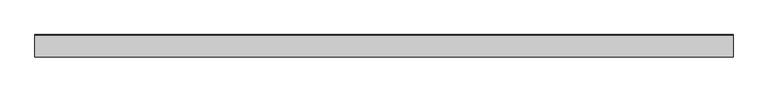
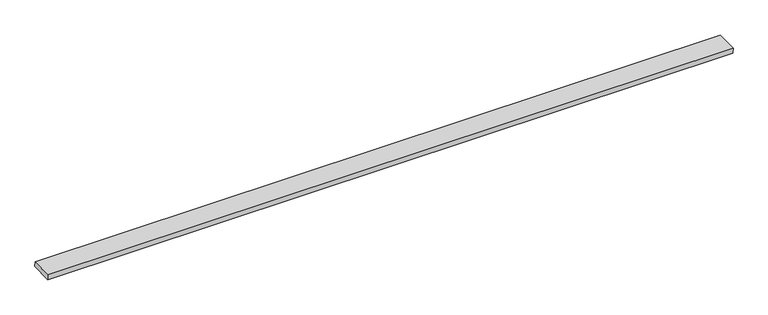
"""IFC4 building model written with IfcOpenShell, lengths in millimetres: proxy geometry, Generic Models 7:Generic Models 1:2:Generic Models 1:2 : Generic Models 7:Generic Models 1:337419:15 : Generic Models 7:Generic Models 1:2:Generic Models 1:2 : Generic Models 7:Generic Models 1:337419:306751."""

from ifc_helpers import new_model, si_unit, frame, origin, place, context, project, spatial, polyline, outline, extrude, source, transform, mapped, element, save


def generic_models_d8c58fdb(model_context):
    return source(origin(), model_context, "Body", "SweptSolid", [
        extrude(outline(polyline([(-578767.7977334, 3680.0317016), (-578769.3002989, 3718.0302757), (-578613.8704771, 3724.5065183), (-578612.3548777, 3686.1783289), (-578767.7977334, 3680.0317016)])), frame((591306.0367239, 0.0, 0.0), z_axis=(1.0, 0.0, 0.0), x_axis=(0.0, 1.0, 0.0)), (0.0, 0.0, 1.0), 4876.8),
    ])


if __name__ == "__main__":
    model = new_model("IFC4")
    model_context = context("Model", 3, world=origin())
    ifc_project = project(units=[si_unit("LENGTHUNIT", "METRE", prefix="MILLI")], contexts=[model_context])
    site = spatial("IfcSite", under=ifc_project)
    building = spatial("IfcBuilding", under=site)
    placement = place(None, origin())
    generic_models_shape = generic_models_d8c58fdb(model_context)
    element("IfcBuildingElementProxy", 1, Name="Generic Models 7:Generic Models 1:2:Generic Models 1:2 : Generic Models 7:Generic Models 1:337419:15 : Generic Models 7:Generic Models 1:2:Generic Models 1:2 : Generic Models 7:Generic Models 1:337419:306751", ObjectType="Generic Models 7:Generic Models 1:2:Generic Models 1:2 : Generic Models 7:Generic Models 1:337419:15 : Generic Models 7:Generic Models 1:2:Generic Models 1:2 : Generic Models 7:Generic Models 1:337419:306751", at=placement, inside=building, context=model_context, shape_type="MappedRepresentation", body=[
        mapped(generic_models_shape, transform((0.0, 0.0, 0.0), x_axis=(1.0, 0.0, 0.0), y_axis=(0.0, 1.0, 0.0), z_axis=(0.0, 0.0, 1.0))),
    ])
    save(model, "model.ifc")

# Revit data of these elements
# Type "Generic Models 7:Generic Models 1:2:Generic Models 1:2 : Generic Models 7:Generic Models 1:337419:15 : Generic Models 7:Generic Models 1:2:Generic Models 1:2 : Generic Models 7:Generic Models 1:337419:306751"
#   NameOverride = "Generic Models 7:Generic Models 1:2:Generic Models 1:2 : Generic Models 7:Generic Models 1:337419:306751"
#   ObjectTypeOverride = "Generic Models 1:2 : Generic Models 7:Generic Models 1:337419"
#   Reference = "Generic Models 1"
#   Tag = "306751"
# Element 1 (IfcBuildingElementProxy, "Generic Models 7:Generic Models 1:2:Generic Models 1:2 : Generic Models 7:Generic Models 1:337419:15 : Generic Models 7:Generic Models 1:2:Generic Models 1:2 : Generic Models 7:Generic Models 1:337419:306751")
#   Materials on its faces: "FIRE RETARDTANT WOOD BLOCKING - SIZE AS NEC."
# Materials
#   "FIRE RETARDTANT WOOD BLOCKING - SIZE AS NEC.": class "Wood", colour RGB 144 113 62, transparency 0, Description = "Pinus Echinata", Cost = 0
